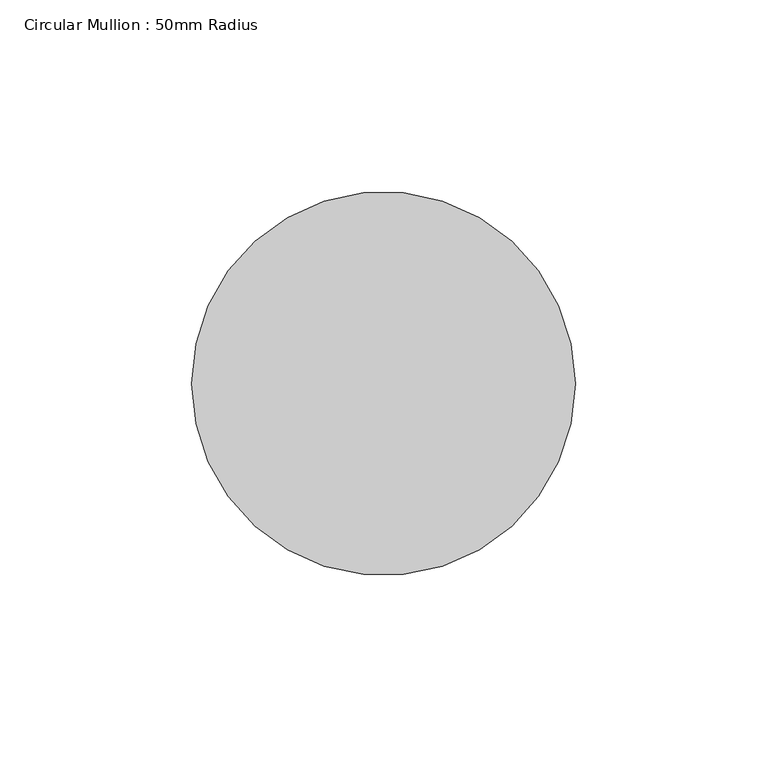
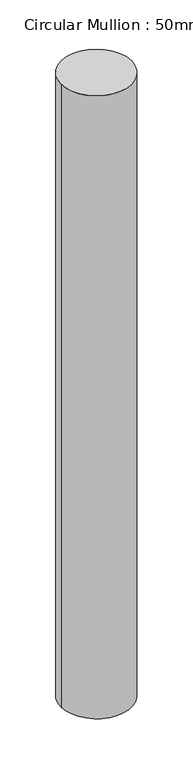
"""IFC4 building model written with IfcOpenShell, lengths in millimetres: member geometry, Circular Mullion : 50mm Radius."""

from ifc_helpers import new_model, si_unit, point, frame, origin, origin_2d, place, context, project, spatial, circle_curve, trimmed, segment, composite_curve, outline, extrude, source, transform, mapped, element, save


def circular_mullion_50mm_radius_6bd68dc3(model_context):
    return source(origin(), model_context, "Body", "SweptSolid", [
        extrude(outline(composite_curve([segment(trimmed(circle_curve(origin_2d(), 50.0), [point((50.0, 0.0))], [point((-50.0, 0.0))], False, "CARTESIAN"), True, "CONTINUOUS"), segment(trimmed(circle_curve(origin_2d(), 50.0), [point((-50.0, 0.0))], [point((50.0, 0.0))], False, "CARTESIAN"), True, "CONTINUOUS")], self_intersect=False)), frame((0.0, 0.0, -934.2913624), z_axis=(0.0, 0.0, 1.0), x_axis=(1.0, 0.0, 0.0)), (0.0, 0.0, 1.0), 934.2913624),
    ])


if __name__ == "__main__":
    model = new_model("IFC4")
    model_context = context("Model", 3, world=origin())
    ifc_project = project(units=[si_unit("LENGTHUNIT", "METRE", prefix="MILLI")], contexts=[model_context])
    site = spatial("IfcSite", under=ifc_project)
    building = spatial("IfcBuilding", under=site)
    placement = place(None, origin())
    circular_mullion_50mm_radius_shape = circular_mullion_50mm_radius_6bd68dc3(model_context)
    element("IfcMember", 1, ObjectType="Circular Mullion : 50mm Radius", at=placement, inside=building, context=model_context, shape_type="MappedRepresentation", body=[
        mapped(circular_mullion_50mm_radius_shape, transform((0.0, 0.0, 0.0), x_axis=(1.0, 0.0, 0.0), y_axis=(0.0, 1.0, 0.0), z_axis=(0.0, 0.0, 1.0))),
    ])
    save(model, "model.ifc")

# Revit data of these elements
# Type "Circular Mullion : 50mm Radius"
#   built-in parameter 1007350 = 0.164042 (stored number, unit not read)
# Element 1 (IfcMember, "Circular Mullion : 50mm Radius")
#   Materials on its faces: "Aluminium"
# Materials
#   "Aluminium": class "Metal", colour RGB 247 247 247, transparency 0, Description = "Aluminium 6061", Cost = 0
